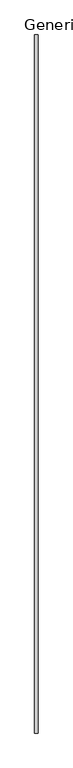
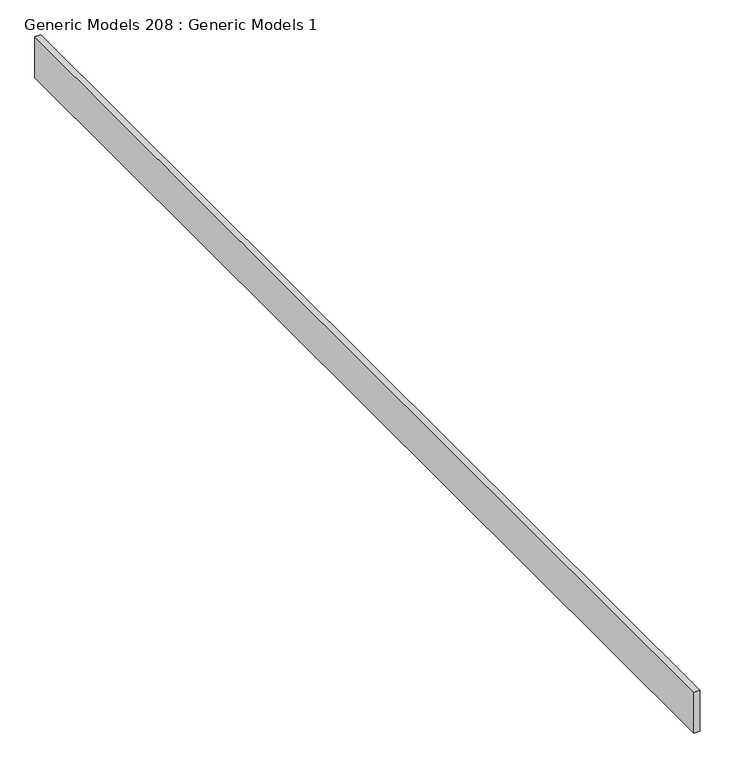
"""IFC4 building model written with IfcOpenShell, lengths in millimetres: proxy geometry, Generic Models 208 : Generic Models 1."""

from ifc_helpers import new_model, si_unit, frame, origin, place, context, project, spatial, polyline, outline, extrude, source, transform, mapped, element, save


def generic_models_208_generic_models_1_8fe7a7c5(model_context):
    return source(origin(), model_context, "Body", "SweptSolid", [
        extrude(outline(polyline([(-8166.2736296, 7054.2769662), (-8128.1736296, 7054.2769662), (-8128.1736296, -464.1230338), (-8166.2736296, -464.1230338), (-8166.2736296, 7054.2769662)])), frame((0.0, 0.0, 126374.271), z_axis=(0.0, 0.0, 1.0), x_axis=(1.0, 0.0, 0.0)), (0.0, 0.0, 1.0), 285.75),
    ])


if __name__ == "__main__":
    model = new_model("IFC4")
    model_context = context("Model", 3, world=origin())
    ifc_project = project(units=[si_unit("LENGTHUNIT", "METRE", prefix="MILLI")], contexts=[model_context])
    site = spatial("IfcSite", under=ifc_project)
    building = spatial("IfcBuilding", under=site)
    placement = place(None, origin())
    generic_models_208_generic_models_1_shape = generic_models_208_generic_models_1_8fe7a7c5(model_context)
    element("IfcBuildingElementProxy", 1, Name="Generic Models 208 : Generic Models 1", ObjectType="Generic Models 208 : Generic Models 1", at=placement, inside=building, context=model_context, shape_type="MappedRepresentation", body=[
        mapped(generic_models_208_generic_models_1_shape, transform((0.0, 0.0, 0.0), x_axis=(1.0, 0.0, 0.0), y_axis=(0.0, 1.0, 0.0), z_axis=(0.0, 0.0, 1.0))),
    ])
    save(model, "model.ifc")

# Revit data of these elements
# Element 1 (IfcBuildingElementProxy, "Generic Models 208 : Generic Models 1")
#   Materials on its faces: "_STRUCTURAL MEMBER (SEE STRUCT. DWGS)"
# Materials
#   "_STRUCTURAL MEMBER (SEE STRUCT. DWGS)": class "Generic", colour RGB 209 182 141, transparency 0, Cost = 0
